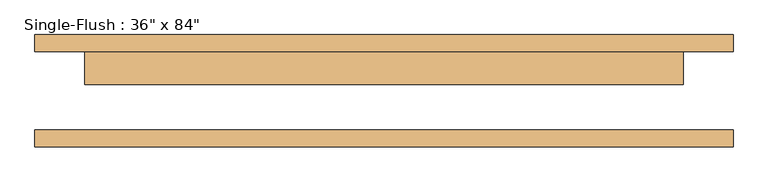
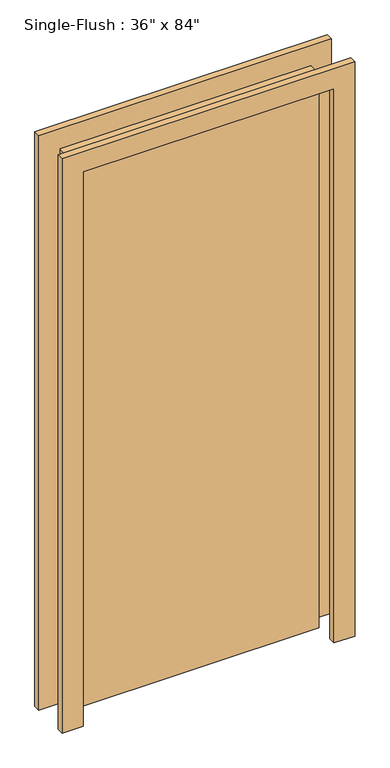
"""IFC4 building model written with IfcOpenShell, lengths in millimetres: door geometry."""

import ifcopenshell
import ifcopenshell.guid

model = None  # the IFC model being written
_history = None  # IfcOwnerHistory: only IFC2X3 demands one
_inside = {}  # id of a spatial element -> (the spatial element, [elements in it])
_under = {}  # id of a project, library or spatial element -> (it, [spatial elements below it])
_declared = {}  # id of a project -> (the project, [libraries it declares])
_typed = {}  # id of a type object -> (the type object, [elements of that type])
_made_of = {}  # id of a material, layer set ... -> (it, [elements and type objects made of it])


def new_model(schema):
    """Start an empty IFC model of exactly this schema.

    Asked for "IFC4X3", IfcOpenShell would pick the latest addendum, in which some entities
    have other attributes; the version numbers below select the first issue.
    IFC2X3 requires an IfcOwnerHistory on every rooted entity: one is made here for all.
    """
    global model, _history
    if schema == "IFC4X3":
        model = ifcopenshell.file(schema_version=(4, 3, 0, 0))
    else:
        model = ifcopenshell.file(schema=schema)
    _inside.clear()
    _under.clear()
    _declared.clear()
    _typed.clear()
    _made_of.clear()
    _history = None
    if model.schema == "IFC2X3":
        org = make("IfcOrganization", Name="unknown")
        user = make(
            "IfcPersonAndOrganization",
            ThePerson=make("IfcPerson", FamilyName="unknown"),
            TheOrganization=org,
        )
        app = make(
            "IfcApplication",
            ApplicationDeveloper=org,
            Version="unknown",
            ApplicationFullName="unknown",
            ApplicationIdentifier="unknown",
        )
        _history = make(
            "IfcOwnerHistory",
            OwningUser=user,
            OwningApplication=app,
            ChangeAction="ADDED",
            CreationDate=0,
        )
    return model


def make(cls, **values):
    """One entity of the class cls with the attributes given. An attribute that is None is left unset."""
    return model.create_entity(
        cls, **{name: value for name, value in values.items() if value is not None}
    )


def rooted(cls, **values):
    """An entity with a GlobalId (a new one), such as an element, a storey or a relation."""
    return make(cls, GlobalId=ifcopenshell.guid.new(), OwnerHistory=_history, **values)


def si_unit(unit_type, name, prefix=None):
    """IfcSIUnit, for example si_unit("LENGTHUNIT", "METRE", prefix="MILLI")."""
    return make("IfcSIUnit", UnitType=unit_type, Prefix=prefix, Name=name)


def assignment(units):
    """IfcUnitAssignment: the units of a project."""
    return None if units is None else make("IfcUnitAssignment", Units=units)


def point(xyz):
    """IfcCartesianPoint."""
    return None if xyz is None else make("IfcCartesianPoint", Coordinates=xyz)


def direction(xyz):
    """IfcDirection."""
    return None if xyz is None else make("IfcDirection", DirectionRatios=xyz)


def frame(location, z_axis=None, x_axis=None):
    """IfcAxis2Placement3D, a coordinate frame: its origin and axes. An axis left out is left unset."""
    return make(
        "IfcAxis2Placement3D",
        Location=point(location),
        Axis=direction(z_axis),
        RefDirection=direction(x_axis),
    )


def origin():
    """The frame at (0, 0, 0) with its axes left unset."""
    return frame((0.0, 0.0, 0.0))


def origin_with_axes():
    """The frame at (0, 0, 0) with the z axis (0, 0, 1) and the x axis (1, 0, 0) written out."""
    return frame((0.0, 0.0, 0.0), z_axis=(0.0, 0.0, 1.0), x_axis=(1.0, 0.0, 0.0))


def place(relative_to, where):
    """IfcLocalPlacement: puts the frame where relative to a parent placement (None: the world)."""
    return make(
        "IfcLocalPlacement", PlacementRelTo=relative_to, RelativePlacement=where
    )


def context(
    kind, dimensions, precision=None, world=None, true_north=None, identifier=None
):
    """IfcGeometricRepresentationContext, for example the 3D "Model" context."""
    return make(
        "IfcGeometricRepresentationContext",
        ContextIdentifier=identifier,
        ContextType=kind,
        CoordinateSpaceDimension=dimensions,
        Precision=precision,
        WorldCoordinateSystem=world,
        TrueNorth=true_north,
    )


def project(units=None, contexts=None):
    """IfcProject with its units and contexts."""
    return rooted(
        "IfcProject",
        Name="project",
        RepresentationContexts=contexts,
        UnitsInContext=assignment(units),
    )


def spatial(cls, under=None, at=None, **own):
    """A site, building, storey or space (cls), placed at a placement, below another one or the project."""
    s = rooted(cls, ObjectPlacement=at, **own)
    if under is not None:
        _under.setdefault(under.id(), (under, []))[1].append(s)
    return s


def polyline(points):
    """IfcPolyline through the points."""
    return make("IfcPolyline", Points=[point(p) for p in points])


def outline(outer, holes=None, kind="AREA"):
    """IfcArbitraryClosedProfileDef: a profile drawn as a closed curve; with holes, ...WithVoids."""
    if holes is None:
        return make("IfcArbitraryClosedProfileDef", ProfileType=kind, OuterCurve=outer)
    return make(
        "IfcArbitraryProfileDefWithVoids",
        ProfileType=kind,
        OuterCurve=outer,
        InnerCurves=holes,
    )


def extrude(swept, where, along, depth):
    """IfcExtrudedAreaSolid: the profile swept, set in the frame where, extruded along a direction by depth."""
    return make(
        "IfcExtrudedAreaSolid",
        SweptArea=swept,
        Position=where,
        ExtrudedDirection=direction(along),
        Depth=depth,
    )


def shape(context_of_items, identifier, shape_type, items):
    """IfcShapeRepresentation: the items that make up one representation, for example the "Body"."""
    return make(
        "IfcShapeRepresentation",
        ContextOfItems=context_of_items,
        RepresentationIdentifier=identifier,
        RepresentationType=shape_type,
        Items=items,
    )


def source(mapping_origin, context_of_items, identifier, shape_type, items):
    """IfcRepresentationMap: a shape defined once, which mapped items show again and again."""
    return make(
        "IfcRepresentationMap",
        MappingOrigin=mapping_origin,
        MappedRepresentation=shape(context_of_items, identifier, shape_type, items),
    )


def transform(
    local_origin,
    x_axis=None,
    y_axis=None,
    z_axis=None,
    scale=None,
    scale2=None,
    scale3=None,
    uniform=True,
):
    """IfcCartesianTransformationOperator3D, or its non-uniform kind. x_axis, y_axis, z_axis: its Axis1, 2, 3."""
    if uniform:
        return make(
            "IfcCartesianTransformationOperator3D",
            Axis1=direction(x_axis),
            Axis2=direction(y_axis),
            LocalOrigin=point(local_origin),
            Scale=scale,
            Axis3=direction(z_axis),
        )
    return make(
        "IfcCartesianTransformationOperator3DnonUniform",
        Axis1=direction(x_axis),
        Axis2=direction(y_axis),
        LocalOrigin=point(local_origin),
        Scale=scale,
        Axis3=direction(z_axis),
        Scale2=scale2,
        Scale3=scale3,
    )


def mapped(mapping_source, mapping_target):
    """IfcMappedItem: shows the shape of a source again, moved by a transform."""
    return make(
        "IfcMappedItem", MappingSource=mapping_source, MappingTarget=mapping_target
    )


def made_of(thing, what):
    """Note that an element or type object is made of a material, layer set ...; save() writes the relation."""
    if what is not None:
        _made_of.setdefault(what.id(), (what, []))[1].append(thing)
    return thing


def element(
    cls,
    number,
    at=None,
    inside=None,
    cuts=None,
    type_object=None,
    material=None,
    context=None,
    identifier="Body",
    shape_type=None,
    held_by="IfcProductDefinitionShape",
    body=None,
    shapes=None,
    **own,
):
    """One element of the class cls, such as IfcWall. Its Tag is "e" and its number.

    at: its placement. inside: the storey or other place that contains it. cuts: it is an
    opening in that element (IfcRelVoidsElement). A single representation is given by context,
    identifier, shape_type and body (its items); several are given by shapes. held_by: the class
    of the entity that holds the representations. save() writes the other relations.
    """
    e = rooted(cls, Tag="e%d" % number, ObjectPlacement=at, **own)
    if body is not None:
        shapes = [shape(context, identifier, shape_type, body)]
    if shapes is not None:
        e.Representation = make(held_by, Representations=shapes)
    if inside is not None:
        _inside.setdefault(inside.id(), (inside, []))[1].append(e)
    if cuts is not None:
        rooted(
            "IfcRelVoidsElement", RelatingBuildingElement=cuts, RelatedOpeningElement=e
        )
    if type_object is not None:
        _typed.setdefault(type_object.id(), (type_object, []))[1].append(e)
    return made_of(e, material)


def aggregate(whole, parts):
    """IfcRelAggregates: a whole, such as a stair, and the parts it consists of."""
    return rooted("IfcRelAggregates", RelatingObject=whole, RelatedObjects=parts)


def save(model, path):
    """Write the relations noted so far, then the file.

    IfcRelAggregates (storeys below a building ...), IfcRelContainedInSpatialStructure (elements
    in a storey), IfcRelDefinesByType, IfcRelAssociatesMaterial and IfcRelDeclares: one each for
    every whole, place, type object, material and project.
    """
    for whole, parts in _under.values():
        aggregate(whole, parts)
    for where, things in _inside.values():
        rooted(
            "IfcRelContainedInSpatialStructure",
            RelatedElements=things,
            RelatingStructure=where,
        )
    for kind, things in _typed.values():
        rooted("IfcRelDefinesByType", RelatedObjects=things, RelatingType=kind)
    for what, things in _made_of.values():
        rooted("IfcRelAssociatesMaterial", RelatedObjects=things, RelatingMaterial=what)
    for by, libraries in _declared.values():
        rooted("IfcRelDeclares", RelatingContext=by, RelatedDefinitions=libraries)
    model.write(path)


def door_aa02eb04(model_context):
    return source(origin(), model_context, "Body", "SweptSolid", [
        extrude(outline(polyline([(2209.8, -533.4), (0.0, -533.4), (0.0, -457.2), (2133.6, -457.2), (2133.6, 457.2), (0.0, 457.2), (0.0, 533.4), (2209.8, 533.4), (2209.8, -533.4)])), frame((0.0, 60.325, 0.0), z_axis=(0.0, 1.0, 0.0), x_axis=(0.0, 0.0, 1.0)), (0.0, 0.0, 1.0), 25.4),
        extrude(outline(polyline([(2209.8, 533.4), (2209.8, -533.4), (0.0, -533.4), (0.0, -457.2), (2133.6, -457.2), (2133.6, 457.2), (0.0, 457.2), (0.0, 533.4), (2209.8, 533.4)])), frame((0.0, -85.725, 0.0), z_axis=(0.0, 1.0, 0.0), x_axis=(0.0, 0.0, 1.0)), (0.0, 0.0, 1.0), 25.4),
        extrude(outline(polyline([(457.2, 9.525), (-457.2, 9.525), (-457.2, 60.325), (457.2, 60.325), (457.2, 9.525)])), origin_with_axes(), (0.0, 0.0, 1.0), 2133.6),
    ])


if __name__ == "__main__":
    model = new_model("IFC4")
    model_context = context("Model", 3, world=origin())
    ifc_project = project(units=[si_unit("LENGTHUNIT", "METRE", prefix="MILLI")], contexts=[model_context])
    site = spatial("IfcSite", under=ifc_project)
    building = spatial("IfcBuilding", under=site)
    placement = place(None, origin())
    door_shape = door_aa02eb04(model_context)
    element("IfcDoor", 1, ObjectType="Single-Flush : 36\" x 84\"", at=placement, inside=building, context=model_context, shape_type="MappedRepresentation", body=[
        mapped(door_shape, transform((0.0, 0.0, 0.0), x_axis=(1.0, 0.0, 0.0), y_axis=(0.0, 1.0, 0.0), z_axis=(0.0, 0.0, 1.0))),
    ])
    save(model, "model.ifc")

# Revit data of these elements
# Type "Single-Flush : 36\" x 84\""
#   Type Mark = "1"
#   Assembly Code = "C1020"
#   Thickness = 0' - 2"
#   Height = 7' - 0"
#   Trim Projection Ext = 0' - 1"
#   Trim Projection Int = 0' - 1"
#   Trim Width = 0' - 3"
#   Width = 3' - 0"
#   Door Material = PAINTED STEEL C CHANNEL
#   Frame Material = PAINTED STEEL C CHANNEL
#   Function = (empty or 0)
#   Wall Closure = (empty or 0)
# Element 1 (IfcDoor, "Single-Flush : 36\" x 84\"")
#   Materials on its faces: "PAINTED STEEL C CHANNEL"
# Materials
#   "PAINTED STEEL C CHANNEL": class "Generic", colour RGB 88 62 61, transparency 0, Cost = 0
